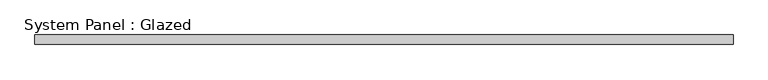
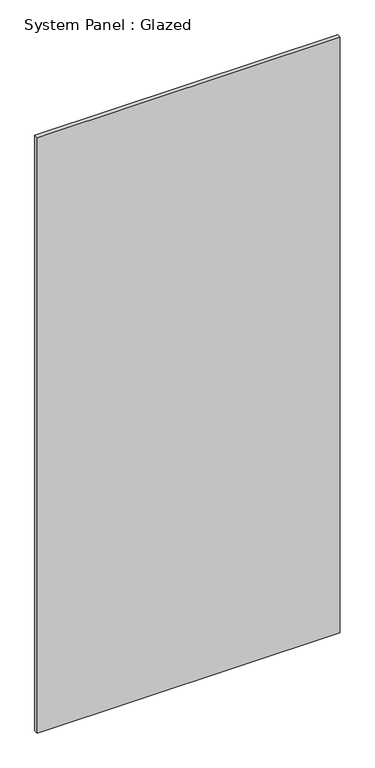
"""IFC4 building model written with IfcOpenShell, lengths in millimetres: plate geometry, System Panel : Glazed."""

from ifc_helpers import new_model, si_unit, origin, origin_with_axes, place, context, project, spatial, polyline, outline, extrude, source, transform, mapped, element, save


def system_panel_glazed_0b61e5af(model_context):
    return source(origin(), model_context, "Body", "SweptSolid", [
        extrude(outline(polyline([(915.0000002, 24.5), (-915.0000002, 24.5), (-915.0000002, 49.5), (915.0000002, 49.5), (915.0000002, 24.5)])), origin_with_axes(), (0.0, 0.0, 1.0), 3800.0),
    ])


if __name__ == "__main__":
    model = new_model("IFC4")
    model_context = context("Model", 3, world=origin())
    ifc_project = project(units=[si_unit("LENGTHUNIT", "METRE", prefix="MILLI")], contexts=[model_context])
    site = spatial("IfcSite", under=ifc_project)
    building = spatial("IfcBuilding", under=site)
    placement = place(None, origin())
    system_panel_glazed_shape = system_panel_glazed_0b61e5af(model_context)
    element("IfcPlate", 1, ObjectType="System Panel : Glazed", at=placement, inside=building, context=model_context, shape_type="MappedRepresentation", body=[
        mapped(system_panel_glazed_shape, transform((0.0, 0.0, 0.0), x_axis=(1.0, 0.0, 0.0), y_axis=(0.0, 1.0, 0.0), z_axis=(0.0, 0.0, 1.0))),
    ])
    save(model, "model.ifc")

# Revit data of these elements
# Type "System Panel : Glazed"
#   Construction Type Id = "GSP4R"
#   Analytic Construction = "1/8 in Pilkington single glazing"
#   Visual Light Transmittance = 0.9
#   Solar Heat Gain Coefficient = 0.86
#   Heat Transfer Coefficient (U) = 6.7069 W/(m²·K)
#   Define Thermal Properties by = 1
# Element 1 (IfcPlate, "System Panel : Glazed")
#   Materials on its faces: "Glass"
# Materials
#   "Glass": class "Glass", colour RGB 0 128 192, transparency 0.9, Description = "Soda Lime Glass", Cost = 0
